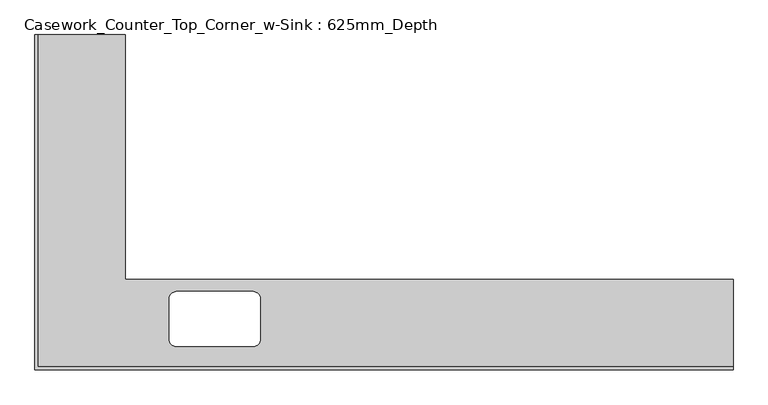
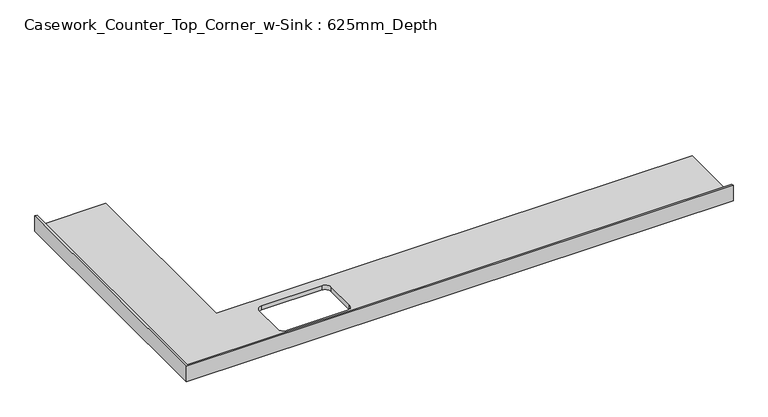
"""IFC4 building model written with IfcOpenShell, lengths in millimetres: furniture geometry, Casework_Counter_Top_Corner_w-Sink : 625mm_Depth."""

from ifc_helpers import new_model, si_unit, frame, origin, place, context, project, spatial, polyline, circle_curve, source, transform, mapped, element, save
from ifc_brep_helpers import plane_surface, revolved_surface, advanced_brep


def casework_counter_top_corner_w_sink_625mm_depth_ef4ba2d1(model_context):
    return source(origin(), model_context, "Body", "AdvancedBrep", [
        advanced_brep(
        [(-575.4622951, 2316.7149096, 900.0), (-1181.4122951, 2316.7149096, 900.0), (-1181.4122951, 19.05, 900.0), (3625.2885505, 19.05, 900.0), (3625.2885505, 625.0, 900.0), (-575.4622951, 625.0, 900.0), (308.4138886, 160.0, 900.0), (-222.7611721, 160.0, 900.0), (-272.7611721, 210.0, 900.0), (-272.7611721, 490.0, 900.0), (-222.7611721, 540.0, 900.0), (308.4138886, 540.0, 900.0), (358.4138886, 490.0, 900.0), (358.4138886, 210.0, 900.0), (3625.2885505, 0.0, 860.0), (-1200.4622951, 0.0, 860.0), (-1200.4622951, 2316.7149096, 860.0), (-575.4622951, 2316.7149096, 860.0), (-575.4622951, 625.0, 860.0), (3625.2885505, 625.0, 860.0), (308.4138886, 160.0, 860.0), (358.4138886, 210.0, 860.0), (358.4138886, 490.0, 860.0), (308.4138886, 540.0, 860.0), (-222.7611721, 540.0, 860.0), (-272.7611721, 490.0, 860.0), (-272.7611721, 210.0, 860.0), (-222.7611721, 160.0, 860.0), (3625.2885505, 0.0, 1001.6), (-1200.4622951, 0.0, 1001.6), (-1200.4622951, 2316.7149096, 1001.6), (-1181.4122951, 2316.7149096, 1001.6), (3625.2885505, 19.05, 1001.6), (-1181.4122951, 19.05, 1001.6)],
        [
            (0, 1),
            (1, 2),
            (2, 3),
            (3, 4),
            (4, 5),
            (5, 0),
            (6, 7),
            (7, 8, circle_curve(frame((-222.7611721, 210.0, 900.0), z_axis=(0.0, 0.0, -1.0), x_axis=(1.0, 0.0, 0.0)), 50.0)),
            (8, 9),
            (9, 10, circle_curve(frame((-222.7611721, 490.0, 900.0), z_axis=(0.0, 0.0, -1.0), x_axis=(1.0, 0.0, 0.0)), 50.0)),
            (10, 11),
            (11, 12, circle_curve(frame((308.4138886, 490.0, 900.0), z_axis=(0.0, 0.0, -1.0), x_axis=(1.0, 0.0, 0.0)), 50.0)),
            (12, 13),
            (13, 6, circle_curve(frame((308.4138886, 210.0, 900.0), z_axis=(0.0, 0.0, -1.0), x_axis=(1.0, 0.0, 0.0)), 50.0)),
            (14, 15),
            (15, 16),
            (16, 17),
            (17, 18),
            (18, 19),
            (19, 14),
            (20, 21, circle_curve(frame((308.4138886, 210.0, 860.0), z_axis=(0.0, 0.0, 1.0), x_axis=(1.0, 0.0, 0.0)), 50.0)),
            (21, 22),
            (22, 23, circle_curve(frame((308.4138886, 490.0, 860.0), z_axis=(0.0, 0.0, 1.0), x_axis=(1.0, 0.0, 0.0)), 50.0)),
            (23, 24),
            (24, 25, circle_curve(frame((-222.7611721, 490.0, 860.0), z_axis=(0.0, 0.0, 1.0), x_axis=(1.0, 0.0, 0.0)), 50.0)),
            (25, 26),
            (26, 27, circle_curve(frame((-222.7611721, 210.0, 860.0), z_axis=(0.0, 0.0, 1.0), x_axis=(1.0, 0.0, 0.0)), 50.0)),
            (27, 20),
            (14, 28),
            (28, 29),
            (29, 15),
            (29, 30),
            (30, 16),
            (30, 31),
            (31, 1),
            (0, 17),
            (5, 18),
            (4, 19),
            (3, 32),
            (32, 28),
            (13, 21),
            (20, 6),
            (12, 22),
            (11, 23),
            (10, 24),
            (9, 25),
            (8, 26),
            (7, 27),
            (32, 33),
            (33, 31),
            (2, 33),
        ],
        [
            plane_surface(frame((-1200.4622951, 0.0, 900.0), z_axis=(0.0, 0.0, 1.0), x_axis=(-1.0, 0.0, 0.0))),
            plane_surface(frame((-1200.4622951, 0.0, 860.0), z_axis=(0.0, 0.0, -1.0), x_axis=(1.0, 0.0, 0.0))),
            plane_surface(frame((3625.2885505, 0.0, 900.0), z_axis=(0.0, -1.0, 0.0), x_axis=(0.0, 0.0, -1.0))),
            plane_surface(frame((-1200.4622951, 0.0, 900.0), z_axis=(-1.0, 0.0, 0.0), x_axis=(0.0, 0.0, -1.0))),
            plane_surface(frame((-1200.4622951, 2316.7149096, 900.0), z_axis=(0.0, 1.0, 0.0), x_axis=(0.0, 0.0, -1.0))),
            plane_surface(frame((-575.4622951, 2316.7149096, 900.0), z_axis=(1.0, 0.0, 0.0), x_axis=(0.0, 0.0, -1.0))),
            plane_surface(frame((-575.4622951, 625.0, 900.0), z_axis=(0.0, 1.0, 0.0), x_axis=(0.0, 0.0, -1.0))),
            plane_surface(frame((3625.2885505, 625.0, 900.0), z_axis=(1.0, 0.0, 0.0), x_axis=(0.0, 0.0, -1.0))),
            revolved_surface(polyline([(358.4138886, 210.0, 860.0), (358.4138886, 210.0, 900.0)]), (308.4138886, 210.0, 0.0), (0.0, 0.0, -1.0)),
            plane_surface(frame((358.4138886, 210.0, 900.0), z_axis=(-1.0, 0.0, 0.0), x_axis=(0.0, 0.0, -1.0))),
            revolved_surface(polyline([(358.4138886, 490.0, 860.0), (358.4138886, 490.0, 900.0)]), (308.4138886, 490.0, 0.0), (0.0, 0.0, -1.0)),
            plane_surface(frame((308.4138886, 540.0, 900.0), z_axis=(0.0, -1.0, 0.0), x_axis=(0.0, 0.0, -1.0))),
            revolved_surface(polyline([(-172.7611721, 490.0, 860.0), (-172.7611721, 490.0, 900.0)]), (-222.7611721, 490.0, 0.0), (0.0, 0.0, -1.0)),
            plane_surface(frame((-272.7611721, 490.0, 900.0), z_axis=(1.0, 0.0, 0.0), x_axis=(0.0, 0.0, -1.0))),
            revolved_surface(polyline([(-172.7611721, 210.0, 860.0), (-172.7611721, 210.0, 900.0)]), (-222.7611721, 210.0, 0.0), (0.0, 0.0, -1.0)),
            plane_surface(frame((-222.7611721, 160.0, 900.0), z_axis=(0.0, 1.0, 0.0), x_axis=(0.0, 0.0, -1.0))),
            plane_surface(frame((-1200.4622951, 0.0, 1001.6), z_axis=(0.0, 0.0, 1.0), x_axis=(0.0, 1.0, 0.0))),
            plane_surface(frame((-1200.4622951, 19.05, 1001.6), z_axis=(0.0, 1.0, 0.0), x_axis=(0.0, 0.0, -1.0))),
            plane_surface(frame((-1181.4122951, 2316.7149096, 1001.6), z_axis=(1.0, 0.0, 0.0), x_axis=(0.0, 0.0, -1.0))),
        ],
        [
            (0, [[1, 2, 3, 4, 5, 6], [7, 8, 9, 10, 11, 12, 13, 14]]),
            (1, [[15, 16, 17, 18, 19, 20], [21, 22, 23, 24, 25, 26, 27, 28]]),
            (2, [[29, 30, 31, -15]]),
            (3, [[-31, 32, 33, -16]]),
            (4, [[34, 35, -1, 36, -17, -33]]),
            (5, [[37, -18, -36, -6]]),
            (6, [[38, -19, -37, -5]]),
            (7, [[-38, -4, 39, 40, -29, -20]]),
            (8, [[41, -21, 42, -14]]),
            (9, [[43, -22, -41, -13]]),
            (10, [[44, -23, -43, -12]]),
            (11, [[45, -24, -44, -11]]),
            (12, [[46, -25, -45, -10]]),
            (13, [[47, -26, -46, -9]]),
            (14, [[48, -27, -47, -8]]),
            (15, [[-42, -28, -48, -7]]),
            (16, [[-30, -40, 49, 50, -34, -32]]),
            (17, [[-3, 51, -49, -39]]),
            (18, [[-51, -2, -35, -50]]),
        ],
    ),
    ])


if __name__ == "__main__":
    model = new_model("IFC4")
    model_context = context("Model", 3, world=origin())
    ifc_project = project(units=[si_unit("LENGTHUNIT", "METRE", prefix="MILLI")], contexts=[model_context])
    site = spatial("IfcSite", under=ifc_project)
    building = spatial("IfcBuilding", under=site)
    placement = place(None, origin())
    casework_counter_top_corner_w_sink_625mm_depth_shape = casework_counter_top_corner_w_sink_625mm_depth_ef4ba2d1(model_context)
    element("IfcFurniture", 1, ObjectType="Casework_Counter_Top_Corner_w-Sink : 625mm_Depth", at=placement, inside=building, context=model_context, shape_type="MappedRepresentation", body=[
        mapped(casework_counter_top_corner_w_sink_625mm_depth_shape, transform((0.0, 0.0, 0.0), x_axis=(1.0, 0.0, 0.0), y_axis=(0.0, 1.0, 0.0), z_axis=(0.0, 0.0, 1.0))),
    ])
    save(model, "model.ifc")

# Revit data of these elements
# Type "Casework_Counter_Top_Corner_w-Sink : 625mm_Depth"
#   Keynote = "N10"
#   Counter Thickness = 40 mm
#   Depth = 625 mm
#   Height = 900 mm
#   Length - Leg 1 [instance default] = 2500 mm
#   Length - Leg 2 [instance default] = 1800 mm
#   Sink Location [instance default] = 1100 mm
#   Sink Location To Wall [instance default] = 160 mm
#   Sink Opening Depth [instance default] = 380 mm
#   Sink Opening Width [instance default] = 690 mm
#   Vis - Worktop Upstand = yes
#   Counter Top Material = Laminate - Marble
# Element 1 (IfcFurniture, "Casework_Counter_Top_Corner_w-Sink : 625mm_Depth")
#   Length - Leg 1 = 4825.751 mm
#   Length - Leg 2 = 2316.715 mm
#   Sink Location = 927.701 mm
#   Sink Opening Width = 631.175 mm
#   Materials on its faces: "Laminate - Marble"
# Materials
#   "Laminate - Marble": class "Miscellaneous", colour RGB 226 177 128, transparency 0
